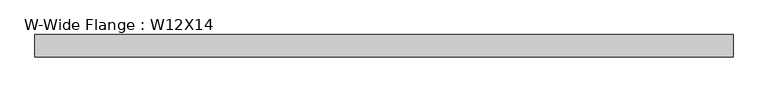
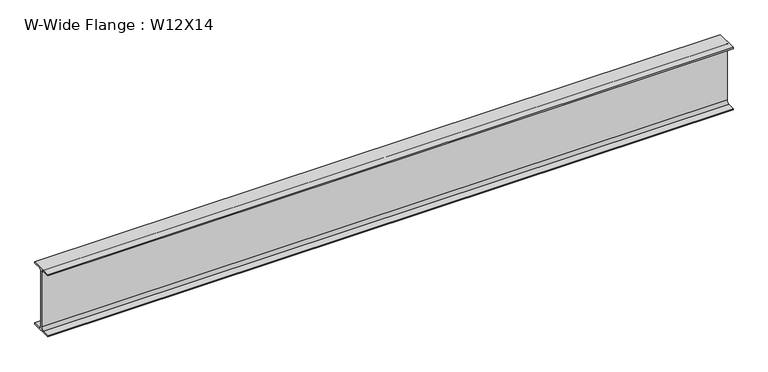
"""IFC4 building model written with IfcOpenShell, lengths in millimetres: beam geometry, W-Wide Flange : W12X14."""

import ifcopenshell
import ifcopenshell.guid

model = None  # the IFC model being written
_history = None  # IfcOwnerHistory: only IFC2X3 demands one
_inside = {}  # id of a spatial element -> (the spatial element, [elements in it])
_under = {}  # id of a project, library or spatial element -> (it, [spatial elements below it])
_declared = {}  # id of a project -> (the project, [libraries it declares])
_typed = {}  # id of a type object -> (the type object, [elements of that type])
_made_of = {}  # id of a material, layer set ... -> (it, [elements and type objects made of it])


def new_model(schema):
    """Start an empty IFC model of exactly this schema.

    Asked for "IFC4X3", IfcOpenShell would pick the latest addendum, in which some entities
    have other attributes; the version numbers below select the first issue.
    IFC2X3 requires an IfcOwnerHistory on every rooted entity: one is made here for all.
    """
    global model, _history
    if schema == "IFC4X3":
        model = ifcopenshell.file(schema_version=(4, 3, 0, 0))
    else:
        model = ifcopenshell.file(schema=schema)
    _inside.clear()
    _under.clear()
    _declared.clear()
    _typed.clear()
    _made_of.clear()
    _history = None
    if model.schema == "IFC2X3":
        org = make("IfcOrganization", Name="unknown")
        user = make(
            "IfcPersonAndOrganization",
            ThePerson=make("IfcPerson", FamilyName="unknown"),
            TheOrganization=org,
        )
        app = make(
            "IfcApplication",
            ApplicationDeveloper=org,
            Version="unknown",
            ApplicationFullName="unknown",
            ApplicationIdentifier="unknown",
        )
        _history = make(
            "IfcOwnerHistory",
            OwningUser=user,
            OwningApplication=app,
            ChangeAction="ADDED",
            CreationDate=0,
        )
    return model


def make(cls, **values):
    """One entity of the class cls with the attributes given. An attribute that is None is left unset."""
    return model.create_entity(
        cls, **{name: value for name, value in values.items() if value is not None}
    )


def rooted(cls, **values):
    """An entity with a GlobalId (a new one), such as an element, a storey or a relation."""
    return make(cls, GlobalId=ifcopenshell.guid.new(), OwnerHistory=_history, **values)


def si_unit(unit_type, name, prefix=None):
    """IfcSIUnit, for example si_unit("LENGTHUNIT", "METRE", prefix="MILLI")."""
    return make("IfcSIUnit", UnitType=unit_type, Prefix=prefix, Name=name)


def assignment(units):
    """IfcUnitAssignment: the units of a project."""
    return None if units is None else make("IfcUnitAssignment", Units=units)


def point(xyz):
    """IfcCartesianPoint."""
    return None if xyz is None else make("IfcCartesianPoint", Coordinates=xyz)


def direction(xyz):
    """IfcDirection."""
    return None if xyz is None else make("IfcDirection", DirectionRatios=xyz)


def frame(location, z_axis=None, x_axis=None):
    """IfcAxis2Placement3D, a coordinate frame: its origin and axes. An axis left out is left unset."""
    return make(
        "IfcAxis2Placement3D",
        Location=point(location),
        Axis=direction(z_axis),
        RefDirection=direction(x_axis),
    )


def frame_2d(location, x_axis=None):
    """IfcAxis2Placement2D, a coordinate frame in the plane: its origin and x axis."""
    return make(
        "IfcAxis2Placement2D", Location=point(location), RefDirection=direction(x_axis)
    )


def origin():
    """The frame at (0, 0, 0) with its axes left unset."""
    return frame((0.0, 0.0, 0.0))


def place(relative_to, where):
    """IfcLocalPlacement: puts the frame where relative to a parent placement (None: the world)."""
    return make(
        "IfcLocalPlacement", PlacementRelTo=relative_to, RelativePlacement=where
    )


def context(
    kind, dimensions, precision=None, world=None, true_north=None, identifier=None
):
    """IfcGeometricRepresentationContext, for example the 3D "Model" context."""
    return make(
        "IfcGeometricRepresentationContext",
        ContextIdentifier=identifier,
        ContextType=kind,
        CoordinateSpaceDimension=dimensions,
        Precision=precision,
        WorldCoordinateSystem=world,
        TrueNorth=true_north,
    )


def project(units=None, contexts=None):
    """IfcProject with its units and contexts."""
    return rooted(
        "IfcProject",
        Name="project",
        RepresentationContexts=contexts,
        UnitsInContext=assignment(units),
    )


def spatial(cls, under=None, at=None, **own):
    """A site, building, storey or space (cls), placed at a placement, below another one or the project."""
    s = rooted(cls, ObjectPlacement=at, **own)
    if under is not None:
        _under.setdefault(under.id(), (under, []))[1].append(s)
    return s


def polyline(points):
    """IfcPolyline through the points."""
    return make("IfcPolyline", Points=[point(p) for p in points])


def circle_curve(where, radius):
    """IfcCircle in the frame where."""
    return make("IfcCircle", Position=where, Radius=radius)


def trimmed(basis, trim1, trim2, sense, master):
    """IfcTrimmedCurve: the piece of a basis curve between two trims."""
    return make(
        "IfcTrimmedCurve",
        BasisCurve=basis,
        Trim1=trim1,
        Trim2=trim2,
        SenseAgreement=sense,
        MasterRepresentation=master,
    )


def segment(curve, same_sense, transition):
    """IfcCompositeCurveSegment."""
    return make(
        "IfcCompositeCurveSegment",
        Transition=transition,
        SameSense=same_sense,
        ParentCurve=curve,
    )


def composite_curve(segments, self_intersect=None):
    """IfcCompositeCurve: segments joined end to end."""
    return make("IfcCompositeCurve", Segments=segments, SelfIntersect=self_intersect)


def outline(outer, holes=None, kind="AREA"):
    """IfcArbitraryClosedProfileDef: a profile drawn as a closed curve; with holes, ...WithVoids."""
    if holes is None:
        return make("IfcArbitraryClosedProfileDef", ProfileType=kind, OuterCurve=outer)
    return make(
        "IfcArbitraryProfileDefWithVoids",
        ProfileType=kind,
        OuterCurve=outer,
        InnerCurves=holes,
    )


def extrude(swept, where, along, depth):
    """IfcExtrudedAreaSolid: the profile swept, set in the frame where, extruded along a direction by depth."""
    return make(
        "IfcExtrudedAreaSolid",
        SweptArea=swept,
        Position=where,
        ExtrudedDirection=direction(along),
        Depth=depth,
    )


def shape(context_of_items, identifier, shape_type, items):
    """IfcShapeRepresentation: the items that make up one representation, for example the "Body"."""
    return make(
        "IfcShapeRepresentation",
        ContextOfItems=context_of_items,
        RepresentationIdentifier=identifier,
        RepresentationType=shape_type,
        Items=items,
    )


def source(mapping_origin, context_of_items, identifier, shape_type, items):
    """IfcRepresentationMap: a shape defined once, which mapped items show again and again."""
    return make(
        "IfcRepresentationMap",
        MappingOrigin=mapping_origin,
        MappedRepresentation=shape(context_of_items, identifier, shape_type, items),
    )


def transform(
    local_origin,
    x_axis=None,
    y_axis=None,
    z_axis=None,
    scale=None,
    scale2=None,
    scale3=None,
    uniform=True,
):
    """IfcCartesianTransformationOperator3D, or its non-uniform kind. x_axis, y_axis, z_axis: its Axis1, 2, 3."""
    if uniform:
        return make(
            "IfcCartesianTransformationOperator3D",
            Axis1=direction(x_axis),
            Axis2=direction(y_axis),
            LocalOrigin=point(local_origin),
            Scale=scale,
            Axis3=direction(z_axis),
        )
    return make(
        "IfcCartesianTransformationOperator3DnonUniform",
        Axis1=direction(x_axis),
        Axis2=direction(y_axis),
        LocalOrigin=point(local_origin),
        Scale=scale,
        Axis3=direction(z_axis),
        Scale2=scale2,
        Scale3=scale3,
    )


def mapped(mapping_source, mapping_target):
    """IfcMappedItem: shows the shape of a source again, moved by a transform."""
    return make(
        "IfcMappedItem", MappingSource=mapping_source, MappingTarget=mapping_target
    )


def made_of(thing, what):
    """Note that an element or type object is made of a material, layer set ...; save() writes the relation."""
    if what is not None:
        _made_of.setdefault(what.id(), (what, []))[1].append(thing)
    return thing


def element(
    cls,
    number,
    at=None,
    inside=None,
    cuts=None,
    type_object=None,
    material=None,
    context=None,
    identifier="Body",
    shape_type=None,
    held_by="IfcProductDefinitionShape",
    body=None,
    shapes=None,
    **own,
):
    """One element of the class cls, such as IfcWall. Its Tag is "e" and its number.

    at: its placement. inside: the storey or other place that contains it. cuts: it is an
    opening in that element (IfcRelVoidsElement). A single representation is given by context,
    identifier, shape_type and body (its items); several are given by shapes. held_by: the class
    of the entity that holds the representations. save() writes the other relations.
    """
    e = rooted(cls, Tag="e%d" % number, ObjectPlacement=at, **own)
    if body is not None:
        shapes = [shape(context, identifier, shape_type, body)]
    if shapes is not None:
        e.Representation = make(held_by, Representations=shapes)
    if inside is not None:
        _inside.setdefault(inside.id(), (inside, []))[1].append(e)
    if cuts is not None:
        rooted(
            "IfcRelVoidsElement", RelatingBuildingElement=cuts, RelatedOpeningElement=e
        )
    if type_object is not None:
        _typed.setdefault(type_object.id(), (type_object, []))[1].append(e)
    return made_of(e, material)


def aggregate(whole, parts):
    """IfcRelAggregates: a whole, such as a stair, and the parts it consists of."""
    return rooted("IfcRelAggregates", RelatingObject=whole, RelatedObjects=parts)


def save(model, path):
    """Write the relations noted so far, then the file.

    IfcRelAggregates (storeys below a building ...), IfcRelContainedInSpatialStructure (elements
    in a storey), IfcRelDefinesByType, IfcRelAssociatesMaterial and IfcRelDeclares: one each for
    every whole, place, type object, material and project.
    """
    for whole, parts in _under.values():
        aggregate(whole, parts)
    for where, things in _inside.values():
        rooted(
            "IfcRelContainedInSpatialStructure",
            RelatedElements=things,
            RelatingStructure=where,
        )
    for kind, things in _typed.values():
        rooted("IfcRelDefinesByType", RelatedObjects=things, RelatingType=kind)
    for what, things in _made_of.values():
        rooted("IfcRelAssociatesMaterial", RelatedObjects=things, RelatingMaterial=what)
    for by, libraries in _declared.values():
        rooted("IfcRelDeclares", RelatingContext=by, RelatedDefinitions=libraries)
    model.write(path)


def w_wide_flange_w12x14_83588449(model_context):
    return source(origin(), model_context, "Body", "SweptSolid", [
        extrude(outline(composite_curve([segment(polyline([(50.419, -145.415), (50.419, -151.13), (-50.419, -151.13), (-50.419, -145.415), (-15.875, -145.415)]), True, "CONTINUOUS"), segment(trimmed(circle_curve(frame_2d((-15.875, -132.08)), 13.335), [point((-15.875, -145.415))], [point((-2.54, -132.08))], True, "CARTESIAN"), True, "CONTINUOUS"), segment(polyline([(-2.54, -132.08), (-2.54, 132.08)]), True, "CONTINUOUS"), segment(trimmed(circle_curve(frame_2d((-15.875, 132.08)), 13.335), [point((-2.54, 132.08))], [point((-15.875, 145.415))], True, "CARTESIAN"), True, "CONTINUOUS"), segment(polyline([(-15.875, 145.415), (-50.419, 145.415), (-50.419, 151.13), (50.419, 151.13), (50.419, 145.415), (15.875, 145.415)]), True, "CONTINUOUS"), segment(trimmed(circle_curve(frame_2d((15.875, 132.08)), 13.335), [point((15.875, 145.415))], [point((2.54, 132.08))], True, "CARTESIAN"), True, "CONTINUOUS"), segment(polyline([(2.54, 132.08), (2.54, -132.08)]), True, "CONTINUOUS"), segment(trimmed(circle_curve(frame_2d((15.875, -132.08)), 13.335), [point((2.54, -132.08))], [point((15.875, -145.415))], True, "CARTESIAN"), True, "CONTINUOUS"), segment(polyline([(15.875, -145.415), (50.419, -145.415)]), True, "CONTINUOUS")], self_intersect=False)), frame((-1574.8, 0.0, 0.0), z_axis=(1.0, 0.0, 0.0), x_axis=(0.0, 1.0, 0.0)), (0.0, 0.0, 1.0), 3149.6),
    ])


if __name__ == "__main__":
    model = new_model("IFC4")
    model_context = context("Model", 3, world=origin())
    ifc_project = project(units=[si_unit("LENGTHUNIT", "METRE", prefix="MILLI")], contexts=[model_context])
    site = spatial("IfcSite", under=ifc_project)
    building = spatial("IfcBuilding", under=site)
    placement = place(None, origin())
    w_wide_flange_w12x14_shape = w_wide_flange_w12x14_83588449(model_context)
    element("IfcBeam", 1, ObjectType="W-Wide Flange : W12X14", at=placement, inside=building, context=model_context, shape_type="MappedRepresentation", body=[
        mapped(w_wide_flange_w12x14_shape, transform((0.0, 0.0, 0.0), x_axis=(1.0, 0.0, 0.0), y_axis=(0.0, 1.0, 0.0), z_axis=(0.0, 0.0, 1.0))),
    ])
    save(model, "model.ifc")

# Revit data of these elements
# Type "W-Wide Flange : W12X14"
#   Assembly Code = "B10"
#   W = 14
#   Length [instance default] = 5' - 0"
#   bf = 0' - 3.97"
#   d = 0' - 11.9"
#   k = 0' - 0 3/4"
#   k2 = 0' - 0.525"
#   tf = 0' - 0.225"
#   tw = 0' - 0.2"
#   A = 0.0288889 SF
#   Structural Material [instance default] = Steel ASTM A992
# Element 1 (IfcBeam, "W-Wide Flange : W12X14")
#   Materials on its faces: "Steel ASTM A992"
# Materials
#   "Steel ASTM A992": class "Metal", colour RGB 199 199 199, transparency 0, Description = "Structural steel 50ksi", Cost = 0
